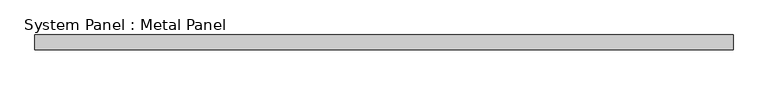
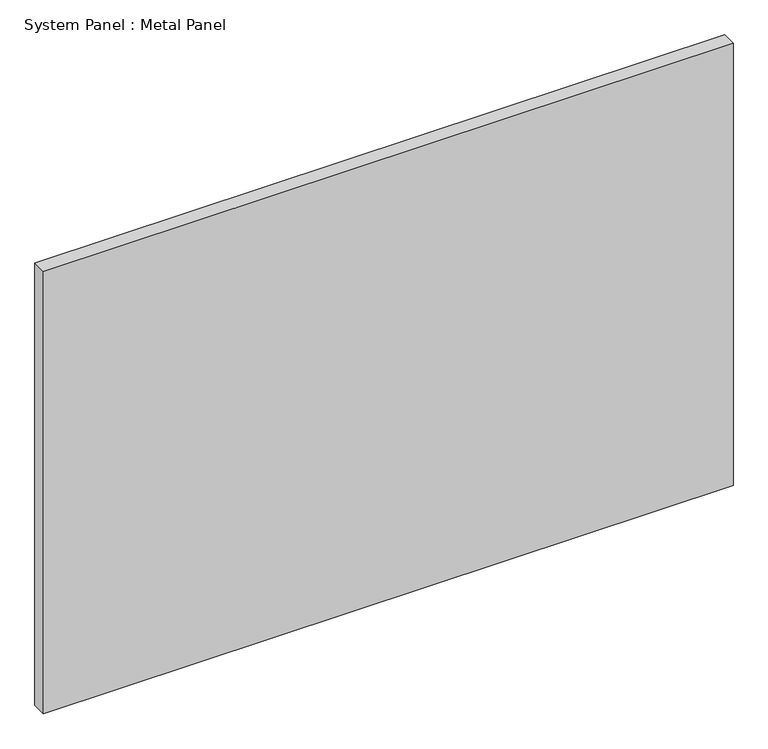
"""IFC4 building model written with IfcOpenShell, lengths in millimetres: plate geometry, System Panel : Metal Panel."""

import ifcopenshell
import ifcopenshell.guid

model = None  # the IFC model being written
_history = None  # IfcOwnerHistory: only IFC2X3 demands one
_inside = {}  # id of a spatial element -> (the spatial element, [elements in it])
_under = {}  # id of a project, library or spatial element -> (it, [spatial elements below it])
_declared = {}  # id of a project -> (the project, [libraries it declares])
_typed = {}  # id of a type object -> (the type object, [elements of that type])
_made_of = {}  # id of a material, layer set ... -> (it, [elements and type objects made of it])


def new_model(schema):
    """Start an empty IFC model of exactly this schema.

    Asked for "IFC4X3", IfcOpenShell would pick the latest addendum, in which some entities
    have other attributes; the version numbers below select the first issue.
    IFC2X3 requires an IfcOwnerHistory on every rooted entity: one is made here for all.
    """
    global model, _history
    if schema == "IFC4X3":
        model = ifcopenshell.file(schema_version=(4, 3, 0, 0))
    else:
        model = ifcopenshell.file(schema=schema)
    _inside.clear()
    _under.clear()
    _declared.clear()
    _typed.clear()
    _made_of.clear()
    _history = None
    if model.schema == "IFC2X3":
        org = make("IfcOrganization", Name="unknown")
        user = make(
            "IfcPersonAndOrganization",
            ThePerson=make("IfcPerson", FamilyName="unknown"),
            TheOrganization=org,
        )
        app = make(
            "IfcApplication",
            ApplicationDeveloper=org,
            Version="unknown",
            ApplicationFullName="unknown",
            ApplicationIdentifier="unknown",
        )
        _history = make(
            "IfcOwnerHistory",
            OwningUser=user,
            OwningApplication=app,
            ChangeAction="ADDED",
            CreationDate=0,
        )
    return model


def make(cls, **values):
    """One entity of the class cls with the attributes given. An attribute that is None is left unset."""
    return model.create_entity(
        cls, **{name: value for name, value in values.items() if value is not None}
    )


def rooted(cls, **values):
    """An entity with a GlobalId (a new one), such as an element, a storey or a relation."""
    return make(cls, GlobalId=ifcopenshell.guid.new(), OwnerHistory=_history, **values)


def si_unit(unit_type, name, prefix=None):
    """IfcSIUnit, for example si_unit("LENGTHUNIT", "METRE", prefix="MILLI")."""
    return make("IfcSIUnit", UnitType=unit_type, Prefix=prefix, Name=name)


def assignment(units):
    """IfcUnitAssignment: the units of a project."""
    return None if units is None else make("IfcUnitAssignment", Units=units)


def point(xyz):
    """IfcCartesianPoint."""
    return None if xyz is None else make("IfcCartesianPoint", Coordinates=xyz)


def direction(xyz):
    """IfcDirection."""
    return None if xyz is None else make("IfcDirection", DirectionRatios=xyz)


def frame(location, z_axis=None, x_axis=None):
    """IfcAxis2Placement3D, a coordinate frame: its origin and axes. An axis left out is left unset."""
    return make(
        "IfcAxis2Placement3D",
        Location=point(location),
        Axis=direction(z_axis),
        RefDirection=direction(x_axis),
    )


def origin():
    """The frame at (0, 0, 0) with its axes left unset."""
    return frame((0.0, 0.0, 0.0))


def origin_with_axes():
    """The frame at (0, 0, 0) with the z axis (0, 0, 1) and the x axis (1, 0, 0) written out."""
    return frame((0.0, 0.0, 0.0), z_axis=(0.0, 0.0, 1.0), x_axis=(1.0, 0.0, 0.0))


def place(relative_to, where):
    """IfcLocalPlacement: puts the frame where relative to a parent placement (None: the world)."""
    return make(
        "IfcLocalPlacement", PlacementRelTo=relative_to, RelativePlacement=where
    )


def context(
    kind, dimensions, precision=None, world=None, true_north=None, identifier=None
):
    """IfcGeometricRepresentationContext, for example the 3D "Model" context."""
    return make(
        "IfcGeometricRepresentationContext",
        ContextIdentifier=identifier,
        ContextType=kind,
        CoordinateSpaceDimension=dimensions,
        Precision=precision,
        WorldCoordinateSystem=world,
        TrueNorth=true_north,
    )


def project(units=None, contexts=None):
    """IfcProject with its units and contexts."""
    return rooted(
        "IfcProject",
        Name="project",
        RepresentationContexts=contexts,
        UnitsInContext=assignment(units),
    )


def spatial(cls, under=None, at=None, **own):
    """A site, building, storey or space (cls), placed at a placement, below another one or the project."""
    s = rooted(cls, ObjectPlacement=at, **own)
    if under is not None:
        _under.setdefault(under.id(), (under, []))[1].append(s)
    return s


def polyline(points):
    """IfcPolyline through the points."""
    return make("IfcPolyline", Points=[point(p) for p in points])


def outline(outer, holes=None, kind="AREA"):
    """IfcArbitraryClosedProfileDef: a profile drawn as a closed curve; with holes, ...WithVoids."""
    if holes is None:
        return make("IfcArbitraryClosedProfileDef", ProfileType=kind, OuterCurve=outer)
    return make(
        "IfcArbitraryProfileDefWithVoids",
        ProfileType=kind,
        OuterCurve=outer,
        InnerCurves=holes,
    )


def extrude(swept, where, along, depth):
    """IfcExtrudedAreaSolid: the profile swept, set in the frame where, extruded along a direction by depth."""
    return make(
        "IfcExtrudedAreaSolid",
        SweptArea=swept,
        Position=where,
        ExtrudedDirection=direction(along),
        Depth=depth,
    )


def shape(context_of_items, identifier, shape_type, items):
    """IfcShapeRepresentation: the items that make up one representation, for example the "Body"."""
    return make(
        "IfcShapeRepresentation",
        ContextOfItems=context_of_items,
        RepresentationIdentifier=identifier,
        RepresentationType=shape_type,
        Items=items,
    )


def source(mapping_origin, context_of_items, identifier, shape_type, items):
    """IfcRepresentationMap: a shape defined once, which mapped items show again and again."""
    return make(
        "IfcRepresentationMap",
        MappingOrigin=mapping_origin,
        MappedRepresentation=shape(context_of_items, identifier, shape_type, items),
    )


def transform(
    local_origin,
    x_axis=None,
    y_axis=None,
    z_axis=None,
    scale=None,
    scale2=None,
    scale3=None,
    uniform=True,
):
    """IfcCartesianTransformationOperator3D, or its non-uniform kind. x_axis, y_axis, z_axis: its Axis1, 2, 3."""
    if uniform:
        return make(
            "IfcCartesianTransformationOperator3D",
            Axis1=direction(x_axis),
            Axis2=direction(y_axis),
            LocalOrigin=point(local_origin),
            Scale=scale,
            Axis3=direction(z_axis),
        )
    return make(
        "IfcCartesianTransformationOperator3DnonUniform",
        Axis1=direction(x_axis),
        Axis2=direction(y_axis),
        LocalOrigin=point(local_origin),
        Scale=scale,
        Axis3=direction(z_axis),
        Scale2=scale2,
        Scale3=scale3,
    )


def mapped(mapping_source, mapping_target):
    """IfcMappedItem: shows the shape of a source again, moved by a transform."""
    return make(
        "IfcMappedItem", MappingSource=mapping_source, MappingTarget=mapping_target
    )


def made_of(thing, what):
    """Note that an element or type object is made of a material, layer set ...; save() writes the relation."""
    if what is not None:
        _made_of.setdefault(what.id(), (what, []))[1].append(thing)
    return thing


def element(
    cls,
    number,
    at=None,
    inside=None,
    cuts=None,
    type_object=None,
    material=None,
    context=None,
    identifier="Body",
    shape_type=None,
    held_by="IfcProductDefinitionShape",
    body=None,
    shapes=None,
    **own,
):
    """One element of the class cls, such as IfcWall. Its Tag is "e" and its number.

    at: its placement. inside: the storey or other place that contains it. cuts: it is an
    opening in that element (IfcRelVoidsElement). A single representation is given by context,
    identifier, shape_type and body (its items); several are given by shapes. held_by: the class
    of the entity that holds the representations. save() writes the other relations.
    """
    e = rooted(cls, Tag="e%d" % number, ObjectPlacement=at, **own)
    if body is not None:
        shapes = [shape(context, identifier, shape_type, body)]
    if shapes is not None:
        e.Representation = make(held_by, Representations=shapes)
    if inside is not None:
        _inside.setdefault(inside.id(), (inside, []))[1].append(e)
    if cuts is not None:
        rooted(
            "IfcRelVoidsElement", RelatingBuildingElement=cuts, RelatedOpeningElement=e
        )
    if type_object is not None:
        _typed.setdefault(type_object.id(), (type_object, []))[1].append(e)
    return made_of(e, material)


def aggregate(whole, parts):
    """IfcRelAggregates: a whole, such as a stair, and the parts it consists of."""
    return rooted("IfcRelAggregates", RelatingObject=whole, RelatedObjects=parts)


def save(model, path):
    """Write the relations noted so far, then the file.

    IfcRelAggregates (storeys below a building ...), IfcRelContainedInSpatialStructure (elements
    in a storey), IfcRelDefinesByType, IfcRelAssociatesMaterial and IfcRelDeclares: one each for
    every whole, place, type object, material and project.
    """
    for whole, parts in _under.values():
        aggregate(whole, parts)
    for where, things in _inside.values():
        rooted(
            "IfcRelContainedInSpatialStructure",
            RelatedElements=things,
            RelatingStructure=where,
        )
    for kind, things in _typed.values():
        rooted("IfcRelDefinesByType", RelatedObjects=things, RelatingType=kind)
    for what, things in _made_of.values():
        rooted("IfcRelAssociatesMaterial", RelatedObjects=things, RelatingMaterial=what)
    for by, libraries in _declared.values():
        rooted("IfcRelDeclares", RelatingContext=by, RelatedDefinitions=libraries)
    model.write(path)


def system_panel_metal_panel_947f48db(model_context):
    return source(origin(), model_context, "Body", "SweptSolid", [
        extrude(outline(polyline([(603.7494819, 19.05), (-603.7494819, 19.05), (-603.7494819, 44.45), (603.7494819, 44.45), (603.7494819, 19.05)])), origin_with_axes(), (0.0, 0.0, 1.0), 819.15),
    ])


if __name__ == "__main__":
    model = new_model("IFC4")
    model_context = context("Model", 3, world=origin())
    ifc_project = project(units=[si_unit("LENGTHUNIT", "METRE", prefix="MILLI")], contexts=[model_context])
    site = spatial("IfcSite", under=ifc_project)
    building = spatial("IfcBuilding", under=site)
    placement = place(None, origin())
    system_panel_metal_panel_shape = system_panel_metal_panel_947f48db(model_context)
    element("IfcPlate", 1, ObjectType="System Panel : Metal Panel", at=placement, inside=building, context=model_context, shape_type="MappedRepresentation", body=[
        mapped(system_panel_metal_panel_shape, transform((0.0, 0.0, 0.0), x_axis=(1.0, 0.0, 0.0), y_axis=(0.0, 1.0, 0.0), z_axis=(0.0, 0.0, 1.0))),
    ])
    save(model, "model.ifc")

# Revit data of these elements
# Element 1 (IfcPlate, "System Panel : Metal Panel")
#   Materials on its faces: "Aluminum"
# Materials
#   "Aluminum": class "Metal", colour RGB 247 247 247, transparency 0, Description = "Aluminum 6061", Cost = 0
